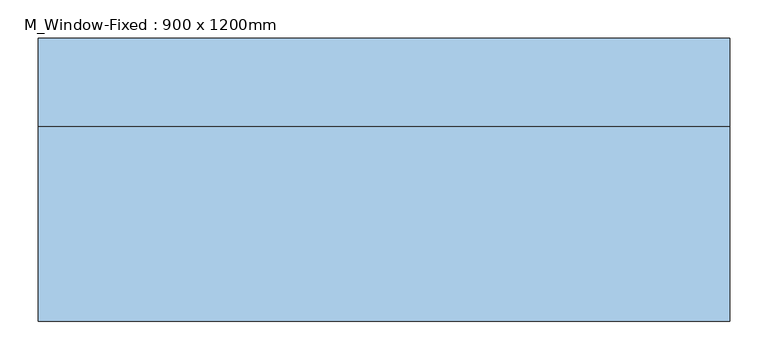
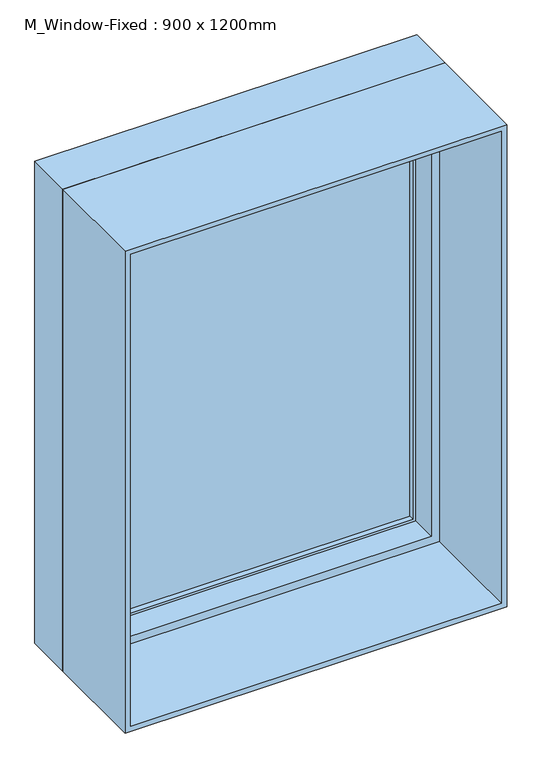
"""IFC4 building model written with IfcOpenShell, lengths in millimetres: window geometry, M_Window-Fixed : 900 x 1200mm."""

from ifc_helpers import new_model, si_unit, frame, origin, place, context, project, spatial, polyline, outline, extrude, faceted_brep, source, transform, mapped, element, save


def m_window_fixed_900_x_1200mm_90fd9cf6(model_context):
    return source(origin(), model_context, "Body", "SolidModel", [
        faceted_brep([(450.0, 79.25, 2100.0), (450.0, 193.55, 2100.0), (-450.0, 193.55, 2100.0), (-450.0, 79.25, 2100.0), (-450.0, 193.55, 900.0), (-450.0, 79.25, 900.0), (450.0, 193.55, 900.0), (450.0, 79.25, 900.0), (418.25, 79.25, 2068.25), (418.25, 79.25, 931.75), (-418.25, 79.25, 931.75), (-418.25, 79.25, 2068.25), (-437.3, 193.55, 2087.3), (-437.3, 193.55, 912.7), (437.3, 193.55, 912.7), (437.3, 193.55, 2087.3), (418.25, 142.75, 2068.25), (-418.25, 142.75, 2068.25), (437.3, 142.75, 2087.3), (-437.3, 142.75, 2087.3), (-418.25, 142.75, 931.75), (-437.3, 142.75, 912.7), (418.25, 142.75, 931.75), (437.3, 142.75, 912.7)], [[[0, 1, 2, 3]], [[3, 2, 4, 5]], [[5, 4, 6, 7]], [[3, 5, 7, 0], [8, 9, 10, 11]], [[7, 6, 1, 0]], [[1, 6, 4, 2], [12, 13, 14, 15]], [[16, 8, 11, 17]], [[15, 18, 19, 12]], [[17, 11, 10, 20]], [[12, 19, 21, 13]], [[20, 10, 9, 22]], [[13, 21, 23, 14]], [[22, 9, 8, 16]], [[18, 23, 21, 19], [17, 20, 22, 16]], [[14, 23, 18, 15]]]),
        extrude(outline(polyline([(2100.0, -450.0), (900.0, -450.0), (900.0, 450.0), (2100.0, 450.0), (2100.0, -450.0)]), holes=[polyline([(2087.3, 437.3), (912.7, 437.3), (912.7, -437.3), (2087.3, -437.3), (2087.3, 437.3)])]), frame((0.0, -174.5, 0.0), z_axis=(0.0, 1.0, 0.0), x_axis=(0.0, 0.0, 1.0)), (0.0, 0.0, 1.0), 253.75),
        extrude(outline(polyline([(912.7, 437.3), (2087.3, 437.3), (2087.3, -437.3), (912.7, -437.3), (912.7, 437.3)]), holes=[polyline([(938.1, -411.9), (2061.9, -411.9), (2061.9, 411.9), (938.1, 411.9), (938.1, -411.9)])]), frame((0.0, 142.75, 0.0), z_axis=(0.0, 1.0, 0.0), x_axis=(0.0, 0.0, 1.0)), (0.0, 0.0, 1.0), 44.45),
        extrude(outline(polyline([(411.9, 174.5), (411.9, 168.15), (-411.9, 168.15), (-411.9, 174.5), (411.9, 174.5)])), frame((0.0, 0.0, 938.1), z_axis=(0.0, 0.0, 1.0), x_axis=(1.0, 0.0, 0.0)), (0.0, 0.0, 1.0), 1123.8),
        extrude(outline(polyline([(-411.9, 155.45), (-411.9, 161.8), (411.9, 161.8), (411.9, 155.45), (-411.9, 155.45)])), frame((0.0, 0.0, 938.1), z_axis=(0.0, 0.0, 1.0), x_axis=(1.0, 0.0, 0.0)), (0.0, 0.0, 1.0), 1123.8),
    ])


if __name__ == "__main__":
    model = new_model("IFC4")
    model_context = context("Model", 3, world=origin())
    ifc_project = project(units=[si_unit("LENGTHUNIT", "METRE", prefix="MILLI")], contexts=[model_context])
    site = spatial("IfcSite", under=ifc_project)
    building = spatial("IfcBuilding", under=site)
    placement = place(None, origin())
    m_window_fixed_900_x_1200mm_shape = m_window_fixed_900_x_1200mm_90fd9cf6(model_context)
    element("IfcWindow", 1, ObjectType="M_Window-Fixed : 900 x 1200mm", at=placement, inside=building, context=model_context, shape_type="MappedRepresentation", body=[
        mapped(m_window_fixed_900_x_1200mm_shape, transform((0.0, 0.0, 0.0), x_axis=(1.0, 0.0, 0.0), y_axis=(0.0, 1.0, 0.0), z_axis=(0.0, 0.0, 1.0))),
    ])
    save(model, "model.ifc")

# Revit data of these elements
# Type "M_Window-Fixed : 900 x 1200mm"
#   Type Mark = "36"
#   Fire Rating = "0.5h"
#   Assembly Code = "B2020100"
#   Analytic Construction = "Double glazing - domestic"
#   Window Inset [instance default] = 0 mm
#   Wall Thickness [instance default] = 150 mm
#   Visual Light Transmittance = 0.81
#   Thermal Resistance (R) = 0.319569 (m²·K)/W
#   Solar Heat Gain Coefficient = 0.76
#   Rough Width = 915 mm
#   Rough Height = 1215 mm
#   Interior Wall Closure [instance default] = 54.75 mm
#   Height = 1200 mm
#   Heat Transfer Coefficient (U) = 3.12929 W/(m²·K)
#   Frame Extension [instance default] = 6.35 mm
#   Exterior Wall Closure [instance default] = 31.75 mm
#   Extension Jamb [instance default] = 54.75 mm
#   Default Sill Height = 900 mm
#   Width = 900 mm
#   Muntin Visibility = yes
#   Interior Trim Visibility [instance default] = yes
#   Exterior Trim Visibility [instance default] = yes
#   Extension Jamb Visibility [instance default] = yes
#   Muntin Pattern = M_Muntin Pattern_2x2 : M_Muntin Pattern_2x2
#   Interior Trim Material = Wood - Stained
#   Interior Trim = M_Trim-Window-Interior-Flat : Picture Frame
#   Interior Frame Material = Wood - Stained
#   Glass Panel Material = Glass
#   Exterior Trim Material = Clad - White
#   Exterior Trim = M_Trim-Window-Exterior-Flat : with Sill
#   Exterior Frame Material = Clad - White
#   Wall Closure = (empty or 0)
# Element 1 (IfcWindow, "M_Window-Fixed : 900 x 1200mm")
#   Wall Thickness = 349 mm
#   Extension Jamb = 253.75 mm
#   Materials on its faces: "Wood - Stained", "Glass", "Clad - White"
# Materials
#   "Wood - Stained": class "Wood", colour RGB 173 132 96, transparency 0, Cost = 0
#   "Glass": class "Glass", colour RGB 245 245 243, transparency 1, Description = "Soda Lime Glass", Cost = 0
#   "Clad - White": class "Wood", colour RGB 245 245 243, transparency 0, Cost = 0
